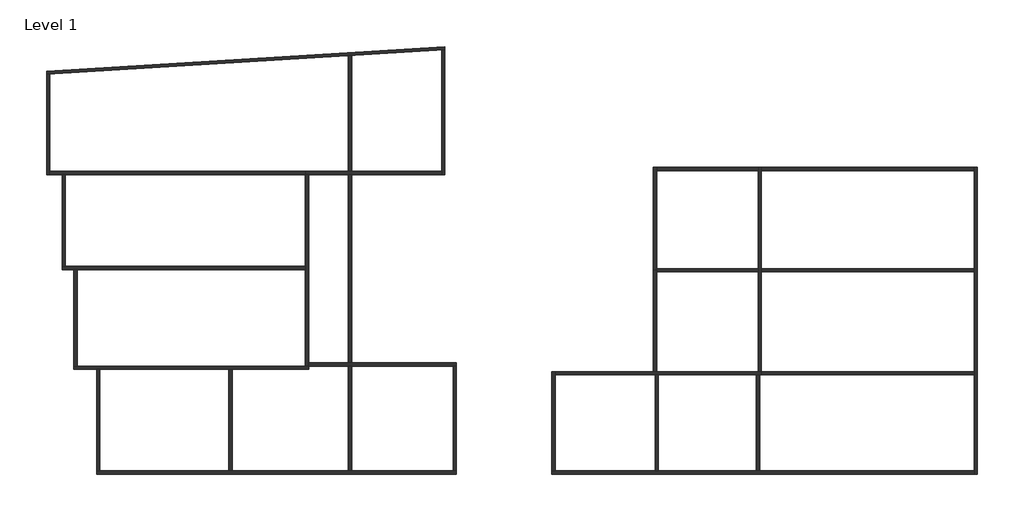
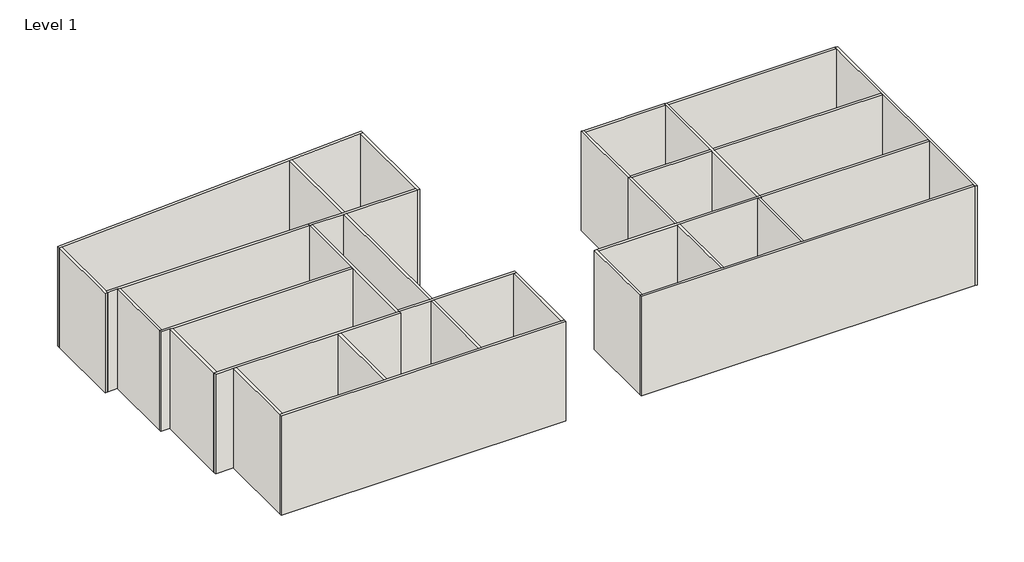
# One storey: 32 walls.
"""IFC4 building model written with IfcOpenShell, lengths in millimetres."""

from ifc_helpers import new_model, si_unit, origin, origin_with_axes, place, context, project, spatial, polyline, outline, extrude, faceted_brep, element, save

model = new_model("IFC4")

# Units and contexts
model_context = context("Model", 3, world=origin())
ifc_project = project(units=[si_unit("LENGTHUNIT", "METRE", prefix="MILLI")], contexts=[model_context])

# Site, building, storey
site = spatial("IfcSite", under=ifc_project)
building = spatial("IfcBuilding", under=site)
storey = spatial("IfcBuildingStorey", under=building, Name="Level 1", Elevation=0.0)

# Walls
placement = place(None, origin())
element("IfcWall", 1, ObjectType="Generic - 200mm", at=placement, inside=storey, context=model_context, shape_type="Brep", body=[
    faceted_brep([(30385.5457783, -10355.6072751, 0.0), (30385.5457783, 8081.1915553, 0.0), (30385.5457783, 8081.1915553, 8000.0), (30385.5457783, -10355.6072751, 8000.0), (30185.5457783, -10355.6072751, 0.0), (30185.5457783, -10355.6072751, 8000.0), (30185.5457783, -10155.6072751, 8000.0), (30185.5457783, -4395.802513, 8000.0), (30185.5457783, -4195.802513, 8000.0), (30185.5457783, 1804.197487, 8000.0), (30185.5457783, 2004.197487, 8000.0), (30185.5457783, 7881.1915553, 8000.0), (30185.5457783, 8081.1915553, 8000.0), (30185.5457783, 8081.1915553, 0.0), (30185.5457783, 7881.1915553, 0.0), (30185.5457783, 2004.197487, 0.0), (30185.5457783, 1804.197487, 0.0), (30185.5457783, -4195.802513, 0.0), (30185.5457783, -4395.802513, 0.0), (30185.5457783, -10155.6072751, 0.0)], [[[0, 1, 2, 3]], [[4, 5, 6, 7, 8, 9, 10, 11, 12, 13, 14, 15, 16, 17, 18, 19]], [[1, 0, 4, 19, 18, 17, 16, 15, 14, 13]], [[3, 2, 12, 11, 10, 9, 8, 7, 6, 5]], [[0, 3, 5, 4]], [[2, 1, 13, 12]]]),
])
element("IfcWall", 2, ObjectType="Generic - 200mm", at=placement, inside=storey, context=model_context, shape_type="Brep", body=[
    faceted_brep([(4799.1027843, -10355.6072751, 0.0), (30185.5457783, -10355.6072751, 0.0), (30185.5457783, -10355.6072751, 8000.0), (4799.1027843, -10355.6072751, 8000.0), (4799.1027843, -10155.6072751, 0.0), (4799.1027843, -10155.6072751, 8000.0), (4999.1027843, -10155.6072751, 8000.0), (10999.1027843, -10155.6072751, 8000.0), (11199.1027843, -10155.6072751, 8000.0), (17099.1027843, -10155.6072751, 8000.0), (17299.1027843, -10155.6072751, 8000.0), (30185.5457783, -10155.6072751, 8000.0), (30185.5457783, -10155.6072751, 0.0), (17299.1027843, -10155.6072751, 0.0), (17099.1027843, -10155.6072751, 0.0), (11199.1027843, -10155.6072751, 0.0), (10999.1027843, -10155.6072751, 0.0), (4999.1027843, -10155.6072751, 0.0)], [[[0, 1, 2, 3]], [[4, 5, 6, 7, 8, 9, 10, 11, 12, 13, 14, 15, 16, 17]], [[1, 0, 4, 17, 16, 15, 14, 13, 12]], [[3, 2, 11, 10, 9, 8, 7, 6, 5]], [[0, 3, 5, 4]], [[2, 1, 12, 11]]]),
])
element("IfcWall", 3, ObjectType="Generic - 200mm", at=placement, inside=storey, context=model_context, shape_type="Brep", body=[
    faceted_brep([(4799.1027843, -4195.802513, 0.0), (4799.1027843, -10155.6072751, 0.0), (4799.1027843, -10155.6072751, 8000.0), (4799.1027843, -4195.802513, 8000.0), (4999.1027843, -4195.802513, 0.0), (4999.1027843, -4195.802513, 8000.0), (4999.1027843, -4395.802513, 8000.0), (4999.1027843, -10155.6072751, 8000.0), (4999.1027843, -10155.6072751, 0.0), (4999.1027843, -4395.802513, 0.0)], [[[0, 1, 2, 3]], [[4, 5, 6, 7, 8, 9]], [[1, 0, 4, 9, 8]], [[3, 2, 7, 6, 5]], [[2, 1, 8, 7]], [[0, 3, 5, 4]]]),
])
element("IfcWall", 4, ObjectType="Generic - 200mm", at=placement, inside=storey, context=model_context, shape_type="Brep", body=[
    faceted_brep([(-25584.210784, 13674.2691465, 0.0), (-25384.210784, 13686.5836155, 0.0), (-7431.0745135, 14792.0003135, 0.0), (-7231.0745135, 14804.3147824, 0.0), (-1831.0745135, 15136.8054448, 0.0), (-1631.0745135, 15149.1199137, 0.0), (-1631.0745135, 15149.1199137, 8000.0), (-1831.0745135, 15136.8054448, 8000.0), (-7231.0745135, 14804.3147824, 8000.0), (-7431.0745135, 14792.0003135, 8000.0), (-25384.210784, 13686.5836155, 8000.0), (-25584.210784, 13674.2691465, 8000.0), (-25584.210784, 13874.6479032, 0.0), (-25584.210784, 13874.6479032, 8000.0), (-1631.0745135, 15349.4986705, 8000.0), (-1631.0745135, 15349.4986705, 0.0)], [[[0, 1, 2, 3, 4, 5, 6, 7, 8, 9, 10, 11]], [[12, 13, 14, 15]], [[5, 4, 3, 2, 1, 0, 12, 15]], [[11, 10, 9, 8, 7, 6, 14, 13]], [[6, 5, 15, 14]], [[0, 11, 13, 12]]]),
])
element("IfcWall", 5, ObjectType="Generic - 200mm", at=placement, inside=storey, context=model_context, shape_type="Brep", body=[
    faceted_brep([(-942.4446045, -10155.6072751, 0.0), (-1142.4446045, -10155.6072751, 0.0), (-7231.0745135, -10155.6072751, 0.0), (-7431.0745135, -10155.6072751, 0.0), (-14431.0745135, -10155.6072751, 0.0), (-14631.0745135, -10155.6072751, 0.0), (-22376.5593682, -10155.6072751, 0.0), (-22576.5593682, -10155.6072751, 0.0), (-22576.5593682, -10155.6072751, 8000.0), (-22376.5593682, -10155.6072751, 8000.0), (-14631.0745135, -10155.6072751, 8000.0), (-14431.0745135, -10155.6072751, 8000.0), (-7431.0745135, -10155.6072751, 8000.0), (-7231.0745135, -10155.6072751, 8000.0), (-1142.4446045, -10155.6072751, 8000.0), (-942.4446045, -10155.6072751, 8000.0), (-942.4446045, -10355.6072751, 0.0), (-942.4446045, -10355.6072751, 8000.0), (-22576.5593682, -10355.6072751, 8000.0), (-22576.5593682, -10355.6072751, 0.0)], [[[0, 1, 2, 3, 4, 5, 6, 7, 8, 9, 10, 11, 12, 13, 14, 15]], [[16, 17, 18, 19]], [[7, 6, 5, 4, 3, 2, 1, 0, 16, 19]], [[15, 14, 13, 12, 11, 10, 9, 8, 18, 17]], [[0, 15, 17, 16]], [[8, 7, 19, 18]]]),
])
element("IfcWall", 6, ObjectType="Generic - 200mm", at=placement, inside=storey, context=model_context, shape_type="Brep", body=[
    faceted_brep([(4999.1027843, -4395.802513, 0.0), (10999.1027843, -4395.802513, 0.0), (11199.1027843, -4395.802513, 0.0), (17099.1027843, -4395.802513, 0.0), (17299.1027843, -4395.802513, 0.0), (17399.1027843, -4395.802513, 0.0), (17399.1027843, -4395.802513, 8000.0), (17299.1027843, -4395.802513, 8000.0), (17099.1027843, -4395.802513, 8000.0), (11199.1027843, -4395.802513, 8000.0), (10999.1027843, -4395.802513, 8000.0), (4999.1027843, -4395.802513, 8000.0), (4999.1027843, -4195.802513, 0.0), (4999.1027843, -4195.802513, 8000.0), (10899.1027843, -4195.802513, 8000.0), (11099.1027843, -4195.802513, 8000.0), (17199.1027843, -4195.802513, 8000.0), (17399.1027843, -4195.802513, 8000.0), (17399.1027843, -4195.802513, 0.0), (17199.1027843, -4195.802513, 0.0), (11099.1027843, -4195.802513, 0.0), (10899.1027843, -4195.802513, 0.0)], [[[0, 1, 2, 3, 4, 5, 6, 7, 8, 9, 10, 11]], [[12, 13, 14, 15, 16, 17, 18, 19, 20, 21]], [[5, 4, 3, 2, 1, 0, 12, 21, 20, 19, 18]], [[11, 10, 9, 8, 7, 6, 17, 16, 15, 14, 13]], [[0, 11, 13, 12]], [[6, 5, 18, 17]]]),
])
element("IfcWall", 7, ObjectType="Generic - 200mm", at=placement, inside=storey, context=model_context, shape_type="Brep", body=[
    faceted_brep([(17399.1027843, -4195.802513, 0.0), (17399.1027843, 1804.197487, 0.0), (17399.1027843, 2004.197487, 0.0), (17399.1027843, 7881.1915553, 0.0), (17399.1027843, 8081.1915553, 0.0), (17399.1027843, 8081.1915553, 8000.0), (17399.1027843, 7881.1915553, 8000.0), (17399.1027843, 2004.197487, 8000.0), (17399.1027843, 1804.197487, 8000.0), (17399.1027843, -4195.802513, 8000.0), (17199.1027843, -4195.802513, 0.0), (17199.1027843, -4195.802513, 8000.0), (17199.1027843, 1804.197487, 8000.0), (17199.1027843, 2004.197487, 8000.0), (17199.1027843, 7881.1915553, 8000.0), (17199.1027843, 8081.1915553, 8000.0), (17199.1027843, 8081.1915553, 0.0), (17199.1027843, 7881.1915553, 0.0), (17199.1027843, 2004.197487, 0.0), (17199.1027843, 1804.197487, 0.0)], [[[0, 1, 2, 3, 4, 5, 6, 7, 8, 9]], [[10, 11, 12, 13, 14, 15, 16, 17, 18, 19]], [[4, 3, 2, 1, 0, 10, 19, 18, 17, 16]], [[9, 8, 7, 6, 5, 15, 14, 13, 12, 11]], [[0, 9, 11, 10]], [[5, 4, 16, 15]]]),
])
element("IfcWall", 8, ObjectType="Generic - 200mm", at=placement, inside=storey, context=model_context, shape_type="SweptSolid", body=[
    extrude(outline(polyline([(30185.5457783, 7881.1915553), (17399.1027843, 7881.1915553), (17399.1027843, 8081.1915553), (30185.5457783, 8081.1915553), (30185.5457783, 7881.1915553)])), origin_with_axes(), (0.0, 0.0, 1.0), 8000.0),
])
element("IfcWall", 9, ObjectType="Generic - 200mm", at=placement, inside=storey, context=model_context, shape_type="Brep", body=[
    faceted_brep([(-1831.0745135, 15136.8054448, 0.0), (-1831.0745135, 7836.8054448, 0.0), (-1831.0745135, 7636.8054448, 0.0), (-1831.0745135, 7636.8054448, 8000.0), (-1831.0745135, 7836.8054448, 8000.0), (-1831.0745135, 15136.8054448, 8000.0), (-1631.0745135, 15149.1199137, 0.0), (-1631.0745135, 15149.1199137, 8000.0), (-1631.0745135, 7636.8054448, 8000.0), (-1631.0745135, 7636.8054448, 0.0)], [[[0, 1, 2, 3, 4, 5]], [[6, 7, 8, 9]], [[2, 1, 0, 6, 9]], [[5, 4, 3, 8, 7]], [[0, 5, 7, 6]], [[3, 2, 9, 8]]]),
])
element("IfcWall", 10, ObjectType="Generic - 200mm", at=placement, inside=storey, context=model_context, shape_type="Brep", body=[
    faceted_brep([(-1831.0745135, 7836.8054448, 0.0), (-7231.0745135, 7836.8054448, 0.0), (-7431.0745135, 7836.8054448, 0.0), (-10031.0745135, 7836.8054448, 0.0), (-10031.0745135, 7836.8054448, 8000.0), (-7431.0745135, 7836.8054448, 8000.0), (-7231.0745135, 7836.8054448, 8000.0), (-1831.0745135, 7836.8054448, 8000.0), (-1831.0745135, 7636.8054448, 0.0), (-1831.0745135, 7636.8054448, 8000.0), (-7231.0745135, 7636.8054448, 8000.0), (-7431.0745135, 7636.8054448, 8000.0), (-9831.0745135, 7636.8054448, 8000.0), (-10031.0745135, 7636.8054448, 8000.0), (-10031.0745135, 7636.8054448, 0.0), (-9831.0745135, 7636.8054448, 0.0), (-7431.0745135, 7636.8054448, 0.0), (-7231.0745135, 7636.8054448, 0.0)], [[[0, 1, 2, 3, 4, 5, 6, 7]], [[8, 9, 10, 11, 12, 13, 14, 15, 16, 17]], [[3, 2, 1, 0, 8, 17, 16, 15, 14]], [[7, 6, 5, 4, 13, 12, 11, 10, 9]], [[0, 7, 9, 8]], [[4, 3, 14, 13]]]),
])
element("IfcWall", 11, ObjectType="Generic - 200mm", at=placement, inside=storey, context=model_context, shape_type="Brep", body=[
    faceted_brep([(-10031.0745135, 7636.8054448, 0.0), (-10031.0745135, 2136.8054448, 0.0), (-10031.0745135, 1936.8054448, 0.0), (-10031.0745135, -3863.1945552, 0.0), (-10031.0745135, -3863.1945552, 8000.0), (-10031.0745135, 1936.8054448, 8000.0), (-10031.0745135, 2136.8054448, 8000.0), (-10031.0745135, 7636.8054448, 8000.0), (-9831.0745135, 7636.8054448, 0.0), (-9831.0745135, 7636.8054448, 8000.0), (-9831.0745135, -3663.1945552, 8000.0), (-9831.0745135, -3863.1945552, 8000.0), (-9831.0745135, -3863.1945552, 0.0), (-9831.0745135, -3663.1945552, 0.0)], [[[0, 1, 2, 3, 4, 5, 6, 7]], [[8, 9, 10, 11, 12, 13]], [[3, 2, 1, 0, 8, 13, 12]], [[7, 6, 5, 4, 11, 10, 9]], [[0, 7, 9, 8]], [[4, 3, 12, 11]]]),
])
element("IfcWall", 12, ObjectType="Generic - 200mm", at=placement, inside=storey, context=model_context, shape_type="Brep", body=[
    faceted_brep([(-9831.0745135, -3863.1945552, 0.0), (-7431.0745135, -3863.1945552, 0.0), (-7231.0745135, -3863.1945552, 0.0), (-1142.4446045, -3863.1945552, 0.0), (-942.4446045, -3863.1945552, 0.0), (-942.4446045, -3863.1945552, 8000.0), (-1142.4446045, -3863.1945552, 8000.0), (-7231.0745135, -3863.1945552, 8000.0), (-7431.0745135, -3863.1945552, 8000.0), (-9831.0745135, -3863.1945552, 8000.0), (-9831.0745135, -3663.1945552, 0.0), (-9831.0745135, -3663.1945552, 8000.0), (-7431.0745135, -3663.1945552, 8000.0), (-7231.0745135, -3663.1945552, 8000.0), (-942.4446045, -3663.1945552, 8000.0), (-942.4446045, -3663.1945552, 0.0), (-7231.0745135, -3663.1945552, 0.0), (-7431.0745135, -3663.1945552, 0.0)], [[[0, 1, 2, 3, 4, 5, 6, 7, 8, 9]], [[10, 11, 12, 13, 14, 15, 16, 17]], [[4, 3, 2, 1, 0, 10, 17, 16, 15]], [[9, 8, 7, 6, 5, 14, 13, 12, 11]], [[0, 9, 11, 10]], [[5, 4, 15, 14]]]),
])
element("IfcWall", 13, ObjectType="Generic - 200mm", at=placement, inside=storey, context=model_context, shape_type="SweptSolid", body=[
    extrude(outline(polyline([(-1142.4446045, -10155.6072751), (-1142.4446045, -3863.1945552), (-942.4446045, -3863.1945552), (-942.4446045, -10155.6072751), (-1142.4446045, -10155.6072751)])), origin_with_axes(), (0.0, 0.0, 1.0), 8000.0),
])
element("IfcWall", 14, ObjectType="Generic - 200mm", at=placement, inside=storey, context=model_context, shape_type="SweptSolid", body=[
    extrude(outline(polyline([(30185.5457783, 1804.197487), (17399.1027843, 1804.197487), (17399.1027843, 2004.197487), (30185.5457783, 2004.197487), (30185.5457783, 1804.197487)])), origin_with_axes(), (0.0, 0.0, 1.0), 8000.0),
])
element("IfcWall", 15, ObjectType="Generic - 200mm", at=placement, inside=storey, context=model_context, shape_type="SweptSolid", body=[
    extrude(outline(polyline([(30185.5457783, -4395.802513), (17399.1027843, -4395.802513), (17399.1027843, -4195.802513), (30185.5457783, -4195.802513), (30185.5457783, -4395.802513)])), origin_with_axes(), (0.0, 0.0, 1.0), 8000.0),
])
element("IfcWall", 16, ObjectType="Generic - 200mm", at=placement, inside=storey, context=model_context, shape_type="SweptSolid", body=[
    extrude(outline(polyline([(10999.1027843, -10155.6072751), (10999.1027843, -4395.802513), (11199.1027843, -4395.802513), (11199.1027843, -10155.6072751), (10999.1027843, -10155.6072751)])), origin_with_axes(), (0.0, 0.0, 1.0), 8000.0),
])
element("IfcWall", 17, ObjectType="Generic - 200mm", at=placement, inside=storey, context=model_context, shape_type="SweptSolid", body=[
    extrude(outline(polyline([(17099.1027843, -10155.6072751), (17099.1027843, -4395.802513), (17299.1027843, -4395.802513), (17299.1027843, -10155.6072751), (17099.1027843, -10155.6072751)])), origin_with_axes(), (0.0, 0.0, 1.0), 8000.0),
])
element("IfcWall", 18, ObjectType="Generic - 200mm", at=placement, inside=storey, context=model_context, shape_type="Brep", body=[
    faceted_brep([(11099.1027843, -4195.802513, 0.0), (11099.1027843, 1804.197487, 0.0), (11099.1027843, 1904.197487, 0.0), (11099.1027843, 1904.197487, 8000.0), (11099.1027843, 1804.197487, 8000.0), (11099.1027843, -4195.802513, 8000.0), (10899.1027843, -4195.802513, 0.0), (10899.1027843, -4195.802513, 8000.0), (10899.1027843, 1904.197487, 8000.0), (10899.1027843, 1904.197487, 0.0)], [[[0, 1, 2, 3, 4, 5]], [[6, 7, 8, 9]], [[2, 1, 0, 6, 9]], [[3, 2, 9, 8]], [[5, 4, 3, 8, 7]], [[0, 5, 7, 6]]]),
])
element("IfcWall", 19, ObjectType="Generic - 200mm", at=placement, inside=storey, context=model_context, shape_type="SweptSolid", body=[
    extrude(outline(polyline([(-7431.0745135, -3663.1945552), (-7431.0745135, 7636.8054448), (-7231.0745135, 7636.8054448), (-7231.0745135, -3663.1945552), (-7431.0745135, -3663.1945552)])), origin_with_axes(), (0.0, 0.0, 1.0), 8000.0),
])
element("IfcWall", 20, ObjectType="Generic - 200mm", at=placement, inside=storey, context=model_context, shape_type="SweptSolid", body=[
    extrude(outline(polyline([(-7231.0745135, 14804.3147824), (-7231.0745135, 7836.8054448), (-7431.0745135, 7836.8054448), (-7431.0745135, 14792.0003135), (-7231.0745135, 14804.3147824)])), origin_with_axes(), (0.0, 0.0, 1.0), 8000.0),
])
element("IfcWall", 21, ObjectType="Generic - 200mm", at=placement, inside=storey, context=model_context, shape_type="Brep", body=[
    faceted_brep([(-10031.0745135, 7836.8054448, 0.0), (-25384.210784, 7836.8054448, 0.0), (-25384.210784, 7836.8054448, 8000.0), (-10031.0745135, 7836.8054448, 8000.0), (-10031.0745135, 7636.8054448, 0.0), (-10031.0745135, 7636.8054448, 8000.0), (-24448.1024259, 7636.8054448, 8000.0), (-24648.1024259, 7636.8054448, 8000.0), (-25384.210784, 7636.8054448, 8000.0), (-25384.210784, 7636.8054448, 0.0), (-24648.1024259, 7636.8054448, 0.0), (-24448.1024259, 7636.8054448, 0.0)], [[[0, 1, 2, 3]], [[4, 5, 6, 7, 8, 9, 10, 11]], [[1, 0, 4, 11, 10, 9]], [[3, 2, 8, 7, 6, 5]], [[0, 3, 5, 4]], [[2, 1, 9, 8]]]),
])
element("IfcWall", 22, ObjectType="Generic - 200mm", at=placement, inside=storey, context=model_context, shape_type="Brep", body=[
    faceted_brep([(-10031.0745135, 2136.8054448, 0.0), (-24448.1024259, 2136.8054448, 0.0), (-24648.1024259, 2136.8054448, 0.0), (-24648.1024259, 2136.8054448, 8000.0), (-24448.1024259, 2136.8054448, 8000.0), (-10031.0745135, 2136.8054448, 8000.0), (-10031.0745135, 1936.8054448, 0.0), (-10031.0745135, 1936.8054448, 8000.0), (-23739.665987, 1936.8054448, 8000.0), (-23939.665987, 1936.8054448, 8000.0), (-24648.1024259, 1936.8054448, 8000.0), (-24648.1024259, 1936.8054448, 0.0), (-23939.665987, 1936.8054448, 0.0), (-23739.665987, 1936.8054448, 0.0)], [[[0, 1, 2, 3, 4, 5]], [[6, 7, 8, 9, 10, 11, 12, 13]], [[2, 1, 0, 6, 13, 12, 11]], [[5, 4, 3, 10, 9, 8, 7]], [[0, 5, 7, 6]], [[3, 2, 11, 10]]]),
])
element("IfcWall", 23, ObjectType="Generic - 200mm", at=placement, inside=storey, context=model_context, shape_type="Brep", body=[
    faceted_brep([(-9831.0745135, -3863.1945552, 0.0), (-23739.665987, -3863.1945552, 0.0), (-23939.665987, -3863.1945552, 0.0), (-23939.665987, -3863.1945552, 8000.0), (-23739.665987, -3863.1945552, 8000.0), (-9831.0745135, -3863.1945552, 8000.0), (-9831.0745135, -4063.1945552, 0.0), (-9831.0745135, -4063.1945552, 8000.0), (-14431.0745135, -4063.1945552, 8000.0), (-14631.0745135, -4063.1945552, 8000.0), (-22376.5593682, -4063.1945552, 8000.0), (-22576.5593682, -4063.1945552, 8000.0), (-23939.665987, -4063.1945552, 8000.0), (-23939.665987, -4063.1945552, 0.0), (-22576.5593682, -4063.1945552, 0.0), (-22376.5593682, -4063.1945552, 0.0), (-14631.0745135, -4063.1945552, 0.0), (-14431.0745135, -4063.1945552, 0.0)], [[[0, 1, 2, 3, 4, 5]], [[6, 7, 8, 9, 10, 11, 12, 13, 14, 15, 16, 17]], [[2, 1, 0, 6, 17, 16, 15, 14, 13]], [[5, 4, 3, 12, 11, 10, 9, 8, 7]], [[0, 5, 7, 6]], [[3, 2, 13, 12]]]),
])
element("IfcWall", 24, ObjectType="Generic - 200mm", at=placement, inside=storey, context=model_context, shape_type="SweptSolid", body=[
    extrude(outline(polyline([(-7431.0745135, -10155.6072751), (-7431.0745135, -3863.1945552), (-7231.0745135, -3863.1945552), (-7231.0745135, -10155.6072751), (-7431.0745135, -10155.6072751)])), origin_with_axes(), (0.0, 0.0, 1.0), 8000.0),
])
element("IfcWall", 25, ObjectType="Generic - 200mm", at=placement, inside=storey, context=model_context, shape_type="SweptSolid", body=[
    extrude(outline(polyline([(-14631.0745135, -10155.6072751), (-14631.0745135, -4063.1945552), (-14431.0745135, -4063.1945552), (-14431.0745135, -10155.6072751), (-14631.0745135, -10155.6072751)])), origin_with_axes(), (0.0, 0.0, 1.0), 8000.0),
])
element("IfcWall", 26, ObjectType="Generic - 200mm", at=placement, inside=storey, context=model_context, shape_type="Brep", body=[
    faceted_brep([(11099.1027843, 1904.197487, 0.0), (11099.1027843, 2004.197487, 0.0), (11099.1027843, 7881.1915553, 0.0), (11099.1027843, 8081.1915553, 0.0), (11099.1027843, 8081.1915553, 8000.0), (11099.1027843, 7881.1915553, 8000.0), (11099.1027843, 2004.197487, 8000.0), (11099.1027843, 1904.197487, 8000.0), (10899.1027843, 1904.197487, 0.0), (10899.1027843, 1904.197487, 8000.0), (10899.1027843, 8081.1915553, 8000.0), (10899.1027843, 8081.1915553, 0.0)], [[[0, 1, 2, 3, 4, 5, 6, 7]], [[8, 9, 10, 11]], [[3, 2, 1, 0, 8, 11]], [[7, 6, 5, 4, 10, 9]], [[0, 7, 9, 8]], [[4, 3, 11, 10]]]),
])
element("IfcWall", 27, ObjectType="Generic - 200mm", at=placement, inside=storey, context=model_context, shape_type="SweptSolid", body=[
    extrude(outline(polyline([(11099.1027843, 8081.1915553), (17199.1027843, 8081.1915553), (17199.1027843, 7881.1915553), (11099.1027843, 7881.1915553), (11099.1027843, 8081.1915553)])), origin_with_axes(), (0.0, 0.0, 1.0), 8000.0),
])
element("IfcWall", 28, ObjectType="Generic - 200mm", at=placement, inside=storey, context=model_context, shape_type="Brep", body=[
    faceted_brep([(17199.1027843, 2004.197487, 0.0), (11099.1027843, 2004.197487, 0.0), (11099.1027843, 2004.197487, 8000.0), (17199.1027843, 2004.197487, 8000.0), (17199.1027843, 1804.197487, 0.0), (17199.1027843, 1804.197487, 8000.0), (11099.1027843, 1804.197487, 8000.0), (11099.1027843, 1804.197487, 0.0), (11099.1027843, 1904.197487, 0.0), (11099.1027843, 1904.197487, 8000.0)], [[[0, 1, 2, 3]], [[4, 5, 6, 7]], [[1, 0, 4, 7, 8]], [[3, 2, 9, 6, 5]], [[2, 1, 8, 7, 6, 9]], [[0, 3, 5, 4]]]),
])
element("IfcWall", 29, ObjectType="Generic - 200mm", at=placement, inside=storey, context=model_context, shape_type="SweptSolid", body=[
    extrude(outline(polyline([(-24448.1024259, 7636.8054448), (-24448.1024259, 2136.8054448), (-24648.1024259, 2136.8054448), (-24648.1024259, 7636.8054448), (-24448.1024259, 7636.8054448)])), origin_with_axes(), (0.0, 0.0, 1.0), 8000.0),
])
element("IfcWall", 30, ObjectType="Generic - 200mm", at=placement, inside=storey, context=model_context, shape_type="Brep", body=[
    faceted_brep([(-25384.210784, 7636.8054448, 0.0), (-25384.210784, 7836.8054448, 0.0), (-25384.210784, 13686.5836155, 0.0), (-25384.210784, 13686.5836155, 8000.0), (-25384.210784, 7836.8054448, 8000.0), (-25384.210784, 7636.8054448, 8000.0), (-25584.210784, 7636.8054448, 0.0), (-25584.210784, 7636.8054448, 8000.0), (-25584.210784, 13674.2691465, 8000.0), (-25584.210784, 13674.2691465, 0.0)], [[[0, 1, 2, 3, 4, 5]], [[6, 7, 8, 9]], [[2, 1, 0, 6, 9]], [[5, 4, 3, 8, 7]], [[3, 2, 9, 8]], [[0, 5, 7, 6]]]),
])
element("IfcWall", 31, ObjectType="Generic - 200mm", at=placement, inside=storey, context=model_context, shape_type="SweptSolid", body=[
    extrude(outline(polyline([(-23739.665987, 1936.8054448), (-23739.665987, -3863.1945552), (-23939.665987, -3863.1945552), (-23939.665987, 1936.8054448), (-23739.665987, 1936.8054448)])), origin_with_axes(), (0.0, 0.0, 1.0), 8000.0),
])
element("IfcWall", 32, ObjectType="Generic - 200mm", at=placement, inside=storey, context=model_context, shape_type="SweptSolid", body=[
    extrude(outline(polyline([(-22376.5593682, -4063.1945552), (-22376.5593682, -10155.6072751), (-22576.5593682, -10155.6072751), (-22576.5593682, -4063.1945552), (-22376.5593682, -4063.1945552)])), origin_with_axes(), (0.0, 0.0, 1.0), 8000.0),
])

save(model, "model.ifc")

# Revit data of these elements
# Project information
#   Project Issue Date = "Issue Date"
#   Project Status = "Project Status"
#   Client Name = "Owner"
#   Project Address = "Enter address here"
#   Project Name = "Project Name"
#   Project Number = "0001"
# Type "Generic - 200mm"
#   Layers, outside or top first: 20 cm no material (function 1)
# Elements 1, 2, 3, 4, 5, 6, 7, 8, 9, 10, 11, 12, 13, 14, 15, 16, 17, 18, 19, 20, 21, 22, 23, 24, 25, 26, 27, 28, 29, 30, 31, 32 (IfcWall, "Generic - 200mm")
#   Top Offset = 0 cm
#   Base Offset = 0 cm
#   Unconnected Height = 800 cm
#   wall height = 800 cm
#   Phase Created = New Construction
#   Base Constraint = Level 1
#   Materials on its faces: "Default Wall"
# Materials
#   "Default Wall": class "Miscellaneous", colour RGB 128 128 128, transparency 0, Cost = 0
# Room at (24755.867, 5541.439) mm, phase "New Construction", upper level "Level 1", upper offset 243.84 cm, lower offset 0 cm
#   Number = "11"
#   Name = "Room"
# Room at (23652.536, -1071.682) mm, phase "New Construction", upper level "Level 1", upper offset 243.84 cm, lower offset 0 cm
#   Number = "12"
#   Name = "Room"
# Room at (23652.536, -7052.899) mm, phase "New Construction", upper level "Level 1", upper offset 243.84 cm, lower offset 0 cm
#   Number = "13"
#   Name = "Room"
# Room, not placed, phase "New Construction", upper offset 0 cm, lower offset 0 cm
#   Number = "14"
#   Name = "Room"
# Room at (7741.338, -7052.899) mm, phase "New Construction", upper level "Level 1", upper offset 243.84 cm, lower offset 0 cm
#   Number = "15"
#   Name = "Room"
# Room at (14535.535, 462.594) mm, phase "New Construction", upper level "Level 1", upper offset 243.84 cm, lower offset 0 cm
#   Number = "16"
#   Name = "Room"
# Room, not placed, phase "New Construction", upper offset 0 cm, lower offset 0 cm
#   Number = "17"
#   Name = "Room"
# Room at (-17285.906, 5082.45) mm, phase "New Construction", upper level "Level 1", upper offset 243.84 cm, lower offset 0 cm
#   Number = "18"
#   Name = "Room"
# Room, not placed, phase "New Construction", upper offset 0 cm, lower offset 0 cm
#   Number = "5"
#   Name = "Room"
# Room, not placed, phase "New Construction", upper offset 0 cm, lower offset 0 cm
#   Number = "6"
#   Name = "Room"
# Room at (-14616.249, 11235.511) mm, phase "New Construction", upper level "Level 1", upper offset 243.84 cm, lower offset 0 cm
#   Number = "9"
#   Name = "Room"
# Room at (-4337.847, 11235.511) mm, phase "New Construction", upper level "Level 1", upper offset 243.84 cm, lower offset 0 cm
#   Number = "10"
#   Name = "Room"
# Area, not placed, upper offset 0 cm, lower offset 0 cm
#   Number = "2"
#   Name = "Area"
# Room, not placed, phase "New Construction", upper offset 0 cm, lower offset 0 cm
#   Number = "1"
#   Name = "Room"
# Area, not placed, upper offset 0 cm, lower offset 0 cm
#   Number = "3"
#   Name = "Area"
# Room at (16426.208, -6054.156) mm, phase "New Construction", upper level "Level 1", upper offset 243.84 cm, lower offset 0 cm
#   Number = "7"
#   Name = "Room"
# Room at (-18664.871, -506.738) mm, phase "New Construction", upper level "Level 1", upper offset 243.84 cm, lower offset 0 cm
#   Number = "8"
#   Name = "Room"
# Room, not placed, phase "New Construction", upper offset 0 cm, lower offset 0 cm
#   Number = "2"
#   Name = "Room"
# Room, not placed, phase "New Construction", upper offset 0 cm, lower offset 0 cm
#   Number = "3"
#   Name = "Room"
# Room, not placed, phase "New Construction", upper offset 0 cm, lower offset 0 cm
#   Number = "4"
#   Name = "Room"
# Area, not placed, upper offset 0 cm, lower offset 0 cm
#   Number = "1"
#   Name = "Area"
